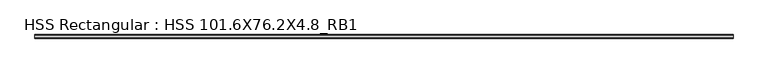
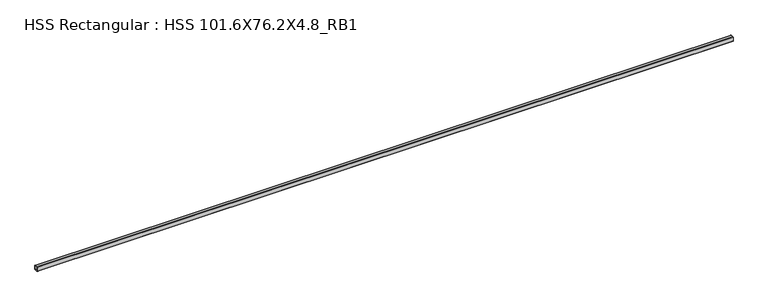
"""IFC4 building model written with IfcOpenShell, lengths in millimetres: beam geometry, HSS Rectangular : HSS 101.6X76.2X4.8_RB1."""

from ifc_helpers import new_model, si_unit, point, frame, frame_2d, origin, place, context, project, spatial, polyline, circle_curve, trimmed, segment, composite_curve, outline, extrude, source, transform, mapped, element, save


def hss_rectangular_hss_101_6x76_2x4_8_rb1_76f34017(model_context):
    return source(origin(), model_context, "Body", "SweptSolid", [
        extrude(outline(composite_curve([segment(polyline([(38.1, 41.275), (38.1, -41.275)]), True, "CONTINUOUS"), segment(trimmed(circle_curve(frame_2d((28.575, -41.275)), 9.525), [point((38.1, -41.275))], [point((28.575, -50.8))], False, "CARTESIAN"), True, "CONTINUOUS"), segment(polyline([(28.575, -50.8), (-28.575, -50.8)]), True, "CONTINUOUS"), segment(trimmed(circle_curve(frame_2d((-28.575, -41.275)), 9.525), [point((-28.575, -50.8))], [point((-38.1, -41.275))], False, "CARTESIAN"), True, "CONTINUOUS"), segment(polyline([(-38.1, -41.275), (-38.1, 41.275)]), True, "CONTINUOUS"), segment(trimmed(circle_curve(frame_2d((-28.575, 41.275)), 9.525), [point((-38.1, 41.275))], [point((-28.575, 50.8))], False, "CARTESIAN"), True, "CONTINUOUS"), segment(polyline([(-28.575, 50.8), (28.575, 50.8)]), True, "CONTINUOUS"), segment(trimmed(circle_curve(frame_2d((28.575, 41.275)), 9.525), [point((28.575, 50.8))], [point((38.1, 41.275))], False, "CARTESIAN"), True, "CONTINUOUS")], self_intersect=False), holes=[composite_curve([segment(trimmed(circle_curve(frame_2d((-28.575, 41.275)), 4.7625), [point((-28.575, 46.0375))], [point((-33.3375, 41.275))], True, "CARTESIAN"), True, "CONTINUOUS"), segment(polyline([(-33.3375, 41.275), (-33.3375, -41.275)]), True, "CONTINUOUS"), segment(trimmed(circle_curve(frame_2d((-28.575, -41.275)), 4.7625), [point((-33.3375, -41.275))], [point((-28.575, -46.0375))], True, "CARTESIAN"), True, "CONTINUOUS"), segment(polyline([(-28.575, -46.0375), (28.575, -46.0375)]), True, "CONTINUOUS"), segment(trimmed(circle_curve(frame_2d((28.575, -41.275)), 4.7625), [point((28.575, -46.0375))], [point((33.3375, -41.275))], True, "CARTESIAN"), True, "CONTINUOUS"), segment(polyline([(33.3375, -41.275), (33.3375, 41.275)]), True, "CONTINUOUS"), segment(trimmed(circle_curve(frame_2d((28.575, 41.275)), 4.7625), [point((33.3375, 41.275))], [point((28.575, 46.0375))], True, "CARTESIAN"), True, "CONTINUOUS"), segment(polyline([(28.575, 46.0375), (-28.575, 46.0375)]), True, "CONTINUOUS")], self_intersect=False)]), frame((-7272.322, 0.0, 0.0), z_axis=(1.0, 0.0, 0.0), x_axis=(0.0, 1.0, 0.0)), (0.0, 0.0, 1.0), 14544.644),
    ])


if __name__ == "__main__":
    model = new_model("IFC4")
    model_context = context("Model", 3, world=origin())
    ifc_project = project(units=[si_unit("LENGTHUNIT", "METRE", prefix="MILLI")], contexts=[model_context])
    site = spatial("IfcSite", under=ifc_project)
    building = spatial("IfcBuilding", under=site)
    placement = place(None, origin())
    hss_rectangular_hss_101_6x76_2x4_8_rb1_shape = hss_rectangular_hss_101_6x76_2x4_8_rb1_76f34017(model_context)
    element("IfcBeam", 1, ObjectType="HSS Rectangular : HSS 101.6X76.2X4.8_RB1", at=placement, inside=building, context=model_context, shape_type="MappedRepresentation", body=[
        mapped(hss_rectangular_hss_101_6x76_2x4_8_rb1_shape, transform((0.0, 0.0, 0.0), x_axis=(1.0, 0.0, 0.0), y_axis=(0.0, 1.0, 0.0), z_axis=(0.0, 0.0, 1.0))),
    ])
    save(model, "model.ifc")

# Revit data of these elements
# Type "HSS Rectangular : HSS 101.6X76.2X4.8_RB1"
#   Section Name Key = "HSS 4X3X3/16"
#   Assembly Code = "B10"
#   Width = 7.62 cm
#   Wall Nominal Thickness = 0.4763 cm
#   Wall Design Thickness = 0.442 cm
#   Torsional Moment of Inertia = 260.561 cm⁴
#   Torsional Modulus = 61.2876 cm³
#   Section Area = 14.4516 cm²
#   Plastic Modulus weak axis = 40.3122 cm³
#   Plastic Modulus strong axis = 49.1612 cm³
#   Perimeter = 0.881482 m²/m
#   Outer Fillet = 0.9525 cm
#   Nominal Weight = 12.1285 kgf/m
#   Moment of Inertia weak axis = 131.529 cm⁴
#   Moment of Inertia strong axis = 205.202 cm⁴
#   Inner Fillet = 0.4763 cm
#   Height = 10.16 cm
#   Elastic Modulus weak axis = 34.4128 cm³
#   Elastic Modulus strong axis = 40.476 cm³
#   Centroid Vertical = 5.08 cm
#   Centroid Horizontal = 3.81 cm
#   Length [instance default] = 1524 mm
#   Structural Material [instance default] = Steel ASTM A500, Grade B, Rectangular and Square
#   Principal Axes Angle = 0
# Element 1 (IfcBeam, "HSS Rectangular : HSS 101.6X76.2X4.8_RB1")
#   Structural Material = Steel ASTM A992
#   Materials on its faces: "Steel ASTM A992"
# Materials
#   "Steel ASTM A500, Grade B, Rectangular and Square": class "Metal", colour RGB 199 199 199, transparency 0, Description = "Carbon steel", Cost = 0
#   "Steel ASTM A992": class "Metal", colour RGB 199 199 199, transparency 0, Description = "Structural steel 50ksi", Cost = 0
